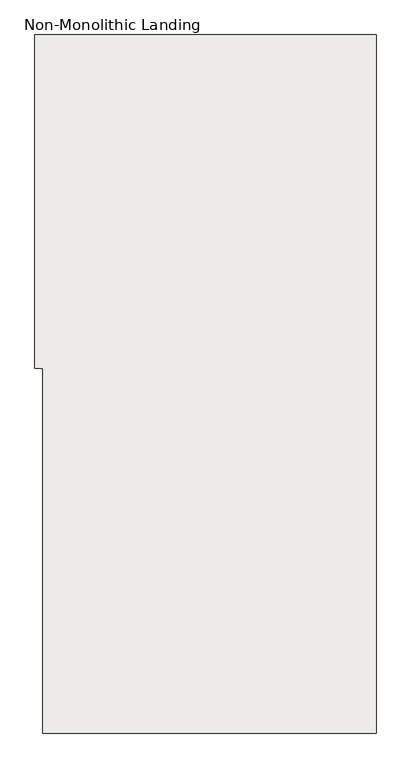
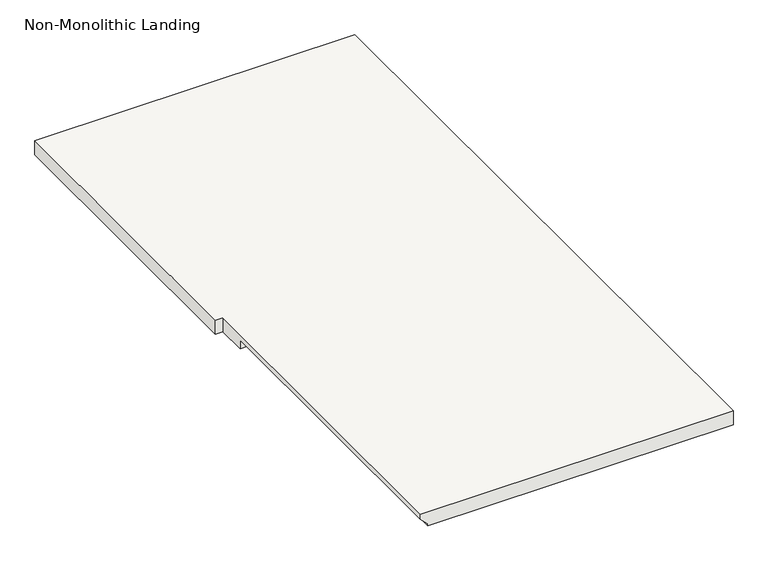
"""IFC4 building model written with IfcOpenShell, lengths in millimetres: slab geometry, Non-Monolithic Landing."""

from ifc_helpers import new_model, si_unit, origin, place, context, project, spatial, faceted_brep, source, transform, mapped, element, save


def non_monolithic_landing_0ff6e51a(model_context):
    return source(origin(), model_context, "Body", "Brep", [
        faceted_brep([(665981.788677, -551651.2413841, 1512.5013514), (665956.388677, -551651.2413841, 1537.9013514), (665956.388677, -550584.4413841, 1537.9013514), (665981.788677, -550584.4413841, 1512.5013514), (667023.188677, -551651.2413841, 1556.9513514), (667023.188677, -549416.0413841, 1556.9513514), (665956.388677, -549416.0413841, 1556.9513514), (665930.988677, -549416.0413841, 1556.9513514), (665930.988677, -550482.8413841, 1556.9513514), (665956.388677, -550482.8413841, 1556.9513514), (665956.388677, -551651.2413841, 1556.9513514), (665981.788677, -550584.4413841, 1506.1513514), (665956.388677, -550584.4413841, 1506.1513514), (665956.388677, -550482.8413841, 1506.1513514), (665930.988677, -550482.8413841, 1506.1513514), (665930.988677, -549416.0413841, 1506.1513514), (665956.388677, -549416.0413841, 1506.1513514), (667023.188677, -549416.0413841, 1506.1513514), (667023.188677, -551651.2413841, 1506.1513514), (665981.788677, -551651.2413841, 1506.1513514)], [[[0, 1, 2, 3]], [[4, 5, 6, 7, 8, 9, 10]], [[11, 12, 13, 14, 15, 16, 17, 18, 19]], [[12, 11, 3, 2]], [[11, 19, 0, 3]], [[4, 10, 1, 0, 19, 18]], [[5, 4, 18, 17]], [[6, 5, 17, 16]], [[7, 6, 16, 15]], [[8, 7, 15, 14]], [[9, 8, 14, 13]], [[10, 9, 13, 12, 2, 1]]]),
    ])


if __name__ == "__main__":
    model = new_model("IFC4")
    model_context = context("Model", 3, world=origin())
    ifc_project = project(units=[si_unit("LENGTHUNIT", "METRE", prefix="MILLI")], contexts=[model_context])
    site = spatial("IfcSite", under=ifc_project)
    building = spatial("IfcBuilding", under=site)
    placement = place(None, origin())
    non_monolithic_landing_shape = non_monolithic_landing_0ff6e51a(model_context)
    element("IfcSlab", 1, ObjectType="Non-Monolithic Landing", at=placement, inside=building, context=model_context, shape_type="MappedRepresentation", body=[
        mapped(non_monolithic_landing_shape, transform((0.0, 0.0, 0.0), x_axis=(1.0, 0.0, 0.0), y_axis=(0.0, 1.0, 0.0), z_axis=(0.0, 0.0, 1.0))),
    ])
    save(model, "model.ifc")
